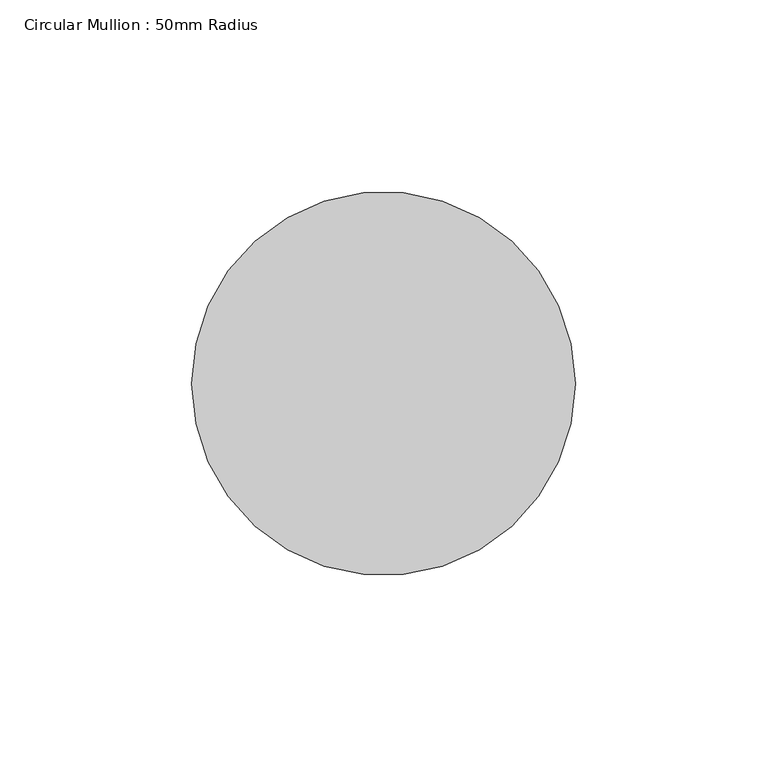
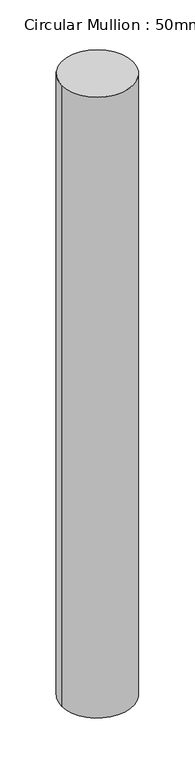
"""IFC4 building model written with IfcOpenShell, lengths in millimetres: member geometry, Circular Mullion : 50mm Radius."""

from ifc_helpers import new_model, si_unit, point, frame, origin, origin_2d, place, context, project, spatial, circle_curve, trimmed, segment, composite_curve, outline, extrude, source, transform, mapped, element, save


def circular_mullion_50mm_radius_2a9faf11(model_context):
    return source(origin(), model_context, "Body", "SweptSolid", [
        extrude(outline(composite_curve([segment(trimmed(circle_curve(origin_2d(), 50.0), [point((50.0, 0.0))], [point((-50.0, 0.0))], False, "CARTESIAN"), True, "CONTINUOUS"), segment(trimmed(circle_curve(origin_2d(), 50.0), [point((-50.0, 0.0))], [point((50.0, 0.0))], False, "CARTESIAN"), True, "CONTINUOUS")], self_intersect=False)), frame((0.0, 0.0, -919.3480517), z_axis=(0.0, 0.0, 1.0), x_axis=(1.0, 0.0, 0.0)), (0.0, 0.0, 1.0), 919.3480517),
    ])


if __name__ == "__main__":
    model = new_model("IFC4")
    model_context = context("Model", 3, world=origin())
    ifc_project = project(units=[si_unit("LENGTHUNIT", "METRE", prefix="MILLI")], contexts=[model_context])
    site = spatial("IfcSite", under=ifc_project)
    building = spatial("IfcBuilding", under=site)
    placement = place(None, origin())
    circular_mullion_50mm_radius_shape = circular_mullion_50mm_radius_2a9faf11(model_context)
    element("IfcMember", 1, ObjectType="Circular Mullion : 50mm Radius", at=placement, inside=building, context=model_context, shape_type="MappedRepresentation", body=[
        mapped(circular_mullion_50mm_radius_shape, transform((0.0, 0.0, 0.0), x_axis=(1.0, 0.0, 0.0), y_axis=(0.0, 1.0, 0.0), z_axis=(0.0, 0.0, 1.0))),
    ])
    save(model, "model.ifc")

# Revit data of these elements
# Type "Circular Mullion : 50mm Radius"
#   built-in parameter 1007350 = 0.164042 (stored number, unit not read)
# Element 1 (IfcMember, "Circular Mullion : 50mm Radius")
#   Materials on its faces: "Aluminium"
# Materials
#   "Aluminium": class "Metal", colour RGB 247 247 247, transparency 0, Description = "Aluminium 6061", Cost = 0
